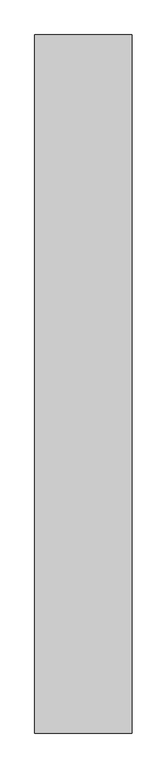
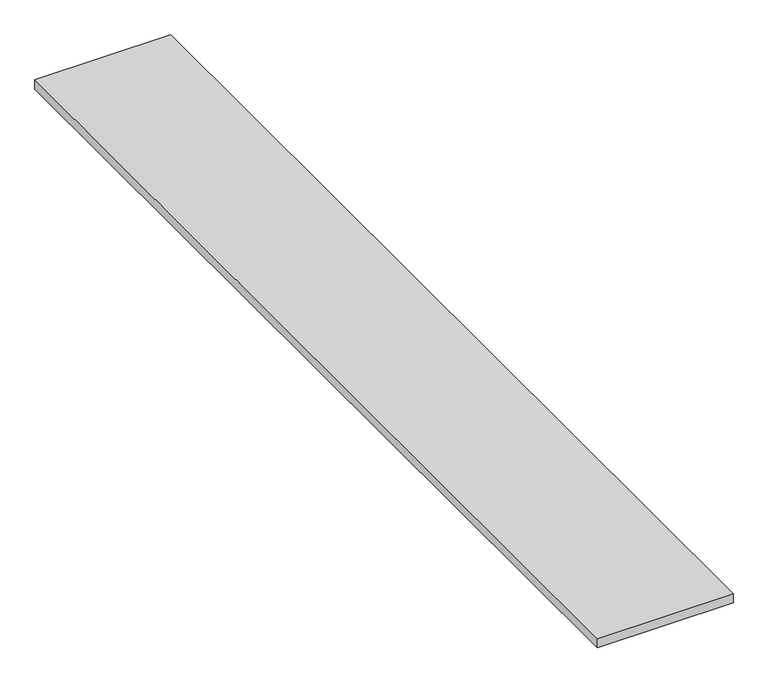
"""IFC4 building model written with IfcOpenShell, lengths in millimetres: furniture geometry, Furniture 4:Furniture 1:2439:Furniture 1:2439 : Furniture 4:Furniture 1:2439:300458 : Furniture 4:Furniture 1:2439:Furniture 1:2439 : Furniture 4:Furniture 1:2439:300458."""

from ifc_helpers import new_model, si_unit, frame, origin, place, context, project, spatial, polyline, outline, extrude, source, transform, mapped, element, save


def furniture_3cdae26c(model_context):
    return source(origin(), model_context, "Body", "SweptSolid", [
        extrude(outline(polyline([(644560.3117239, -570612.3413841), (644204.7117239, -570612.3413841), (644204.7117239, -568059.6413841), (644560.3117239, -568059.6413841), (644560.3117239, -570612.3413841)])), frame((0.0, 0.0, 381.0), z_axis=(0.0, 0.0, 1.0), x_axis=(1.0, 0.0, 0.0)), (0.0, 0.0, 1.0), 25.4),
    ])


if __name__ == "__main__":
    model = new_model("IFC4")
    model_context = context("Model", 3, world=origin())
    ifc_project = project(units=[si_unit("LENGTHUNIT", "METRE", prefix="MILLI")], contexts=[model_context])
    site = spatial("IfcSite", under=ifc_project)
    building = spatial("IfcBuilding", under=site)
    placement = place(None, origin())
    furniture_shape = furniture_3cdae26c(model_context)
    element("IfcFurniture", 1, ObjectType="Furniture 4:Furniture 1:2439:Furniture 1:2439 : Furniture 4:Furniture 1:2439:300458 : Furniture 4:Furniture 1:2439:Furniture 1:2439 : Furniture 4:Furniture 1:2439:300458", at=placement, inside=building, context=model_context, shape_type="MappedRepresentation", body=[
        mapped(furniture_shape, transform((0.0, 0.0, 0.0), x_axis=(1.0, 0.0, 0.0), y_axis=(0.0, 1.0, 0.0), z_axis=(0.0, 0.0, 1.0))),
    ])
    save(model, "model.ifc")

# Revit data of these elements
# Type "Furniture 4:Furniture 1:2439:Furniture 1:2439 : Furniture 4:Furniture 1:2439:300458 : Furniture 4:Furniture 1:2439:Furniture 1:2439 : Furniture 4:Furniture 1:2439:300458"
#   NameOverride = "Furniture 4:Furniture 1:2439:Furniture 1:2439 : Furniture 4:Furniture 1:2439:300458"
#   ObjectTypeOverride = "Furniture 1:2439 : Furniture 4:Furniture 1:2439"
#   Tag = "300458"
